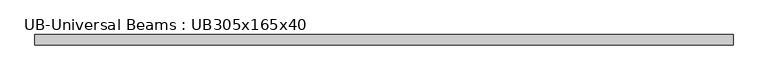
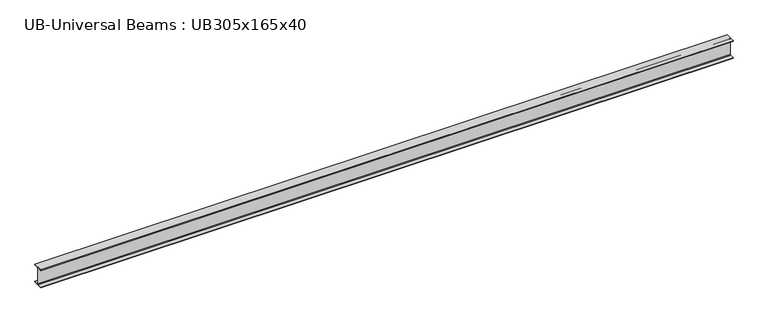
"""IFC4 building model written with IfcOpenShell, lengths in millimetres: member geometry, UB-Universal Beams : UB305x165x40."""

from ifc_helpers import new_model, si_unit, point, frame, frame_2d, origin, place, context, project, spatial, polyline, circle_curve, trimmed, segment, composite_curve, outline, extrude, source, transform, mapped, element, save


def ub_universal_beams_ub305x165x40_8d2bc380(model_context):
    return source(origin(), model_context, "Body", "SweptSolid", [
        extrude(outline(composite_curve([segment(polyline([(82.5, -141.5), (82.5, -151.7), (-82.5, -151.7), (-82.5, -141.5), (-11.9, -141.5)]), True, "CONTINUOUS"), segment(trimmed(circle_curve(frame_2d((-11.9, -132.6)), 8.9), [point((-11.9, -141.5))], [point((-3.0, -132.6))], True, "CARTESIAN"), True, "CONTINUOUS"), segment(polyline([(-3.0, -132.6), (-3.0, 132.6)]), True, "CONTINUOUS"), segment(trimmed(circle_curve(frame_2d((-11.9, 132.6)), 8.9), [point((-3.0, 132.6))], [point((-11.9, 141.5))], True, "CARTESIAN"), True, "CONTINUOUS"), segment(polyline([(-11.9, 141.5), (-82.5, 141.5), (-82.5, 151.7), (82.5, 151.7), (82.5, 141.5), (11.9, 141.5)]), True, "CONTINUOUS"), segment(trimmed(circle_curve(frame_2d((11.9, 132.6)), 8.9), [point((11.9, 141.5))], [point((3.0, 132.6))], True, "CARTESIAN"), True, "CONTINUOUS"), segment(polyline([(3.0, 132.6), (3.0, -132.6)]), True, "CONTINUOUS"), segment(trimmed(circle_curve(frame_2d((11.9, -132.6)), 8.9), [point((3.0, -132.6))], [point((11.9, -141.5))], True, "CARTESIAN"), True, "CONTINUOUS"), segment(polyline([(11.9, -141.5), (82.5, -141.5)]), True, "CONTINUOUS")], self_intersect=False)), frame((-5621.7, 0.0, 0.0), z_axis=(1.0, 0.0, 0.0), x_axis=(0.0, 1.0, 0.0)), (0.0, 0.0, 1.0), 11256.5),
    ])


if __name__ == "__main__":
    model = new_model("IFC4")
    model_context = context("Model", 3, world=origin())
    ifc_project = project(units=[si_unit("LENGTHUNIT", "METRE", prefix="MILLI")], contexts=[model_context])
    site = spatial("IfcSite", under=ifc_project)
    building = spatial("IfcBuilding", under=site)
    placement = place(None, origin())
    ub_universal_beams_ub305x165x40_shape = ub_universal_beams_ub305x165x40_8d2bc380(model_context)
    element("IfcMember", 1, ObjectType="UB-Universal Beams : UB305x165x40", at=placement, inside=building, context=model_context, shape_type="MappedRepresentation", body=[
        mapped(ub_universal_beams_ub305x165x40_shape, transform((0.0, 0.0, 0.0), x_axis=(1.0, 0.0, 0.0), y_axis=(0.0, 1.0, 0.0), z_axis=(0.0, 0.0, 1.0))),
    ])
    save(model, "model.ifc")

# Revit data of these elements
# Type "UB-Universal Beams : UB305x165x40"
#   Section Name Key = "UB305X165X40"
#   Width = 16.5 cm
#   Web Thickness = 0.6 cm
#   Web Fillet = 0.89 cm
#   Warping Constant = 164000.0 cm⁶
#   Torsional Moment of Inertia = 14.70 cm⁴
#   Section Area = 51.3 cm²
#   Plastic Modulus weak axis = 142.0 cm³
#   Plastic Modulus strong axis = 623.0 cm³
#   Nominal Weight = 40.2999 kgf/m
#   Moment of Inertia weak axis = 764.00 cm⁴
#   Moment of Inertia strong axis = 8503.00 cm⁴
#   Height = 30.34 cm
#   Flange Thickness = 1.02 cm
#   Elastic Modulus weak axis = 92.6 cm³
#   Elastic Modulus strong axis = 560.0 cm³
#   Centroid Vertical = 15.17 cm
#   Centroid Horizontal = 8.25 cm
#   Bolt Spacing = 9.0 cm
#   Length [instance default] = 1500 mm
#   Structural Material [instance default] = Metal - Steel 43-275
#   Type Comments = ""
#   Assembly Code = ""
# Element 1 (IfcMember, "UB-Universal Beams : UB305x165x40")
#   Materials on its faces: "Metal - Steel 43-275"
# Materials
#   "Metal - Steel 43-275": class "Metal", colour RGB 247 247 247, transparency 0, Cost = 0
